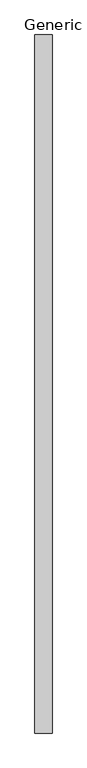
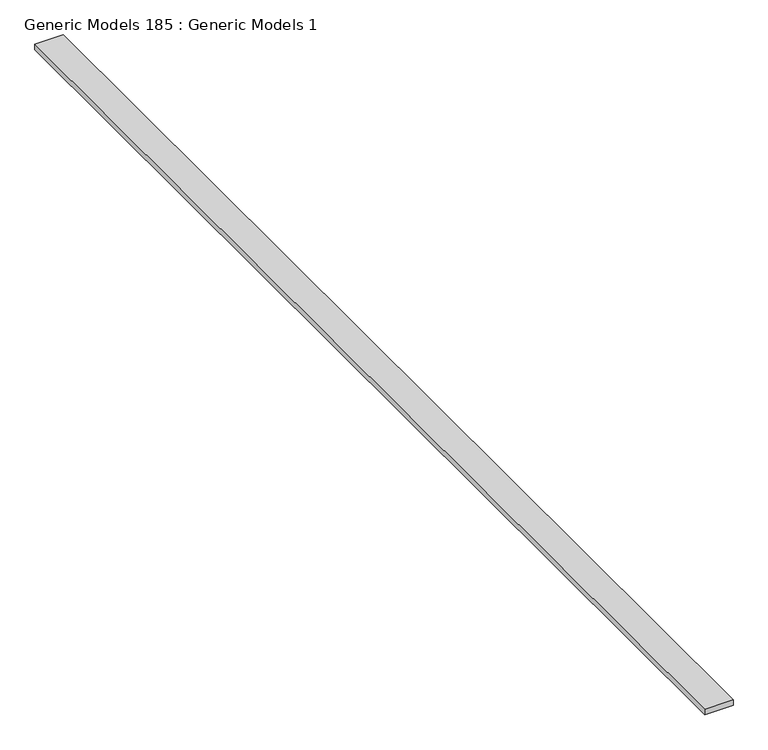
"""IFC4 building model written with IfcOpenShell, lengths in millimetres: proxy geometry, Generic Models 185 : Generic Models 1."""

import ifcopenshell
import ifcopenshell.guid

model = None  # the IFC model being written
_history = None  # IfcOwnerHistory: only IFC2X3 demands one
_inside = {}  # id of a spatial element -> (the spatial element, [elements in it])
_under = {}  # id of a project, library or spatial element -> (it, [spatial elements below it])
_declared = {}  # id of a project -> (the project, [libraries it declares])
_typed = {}  # id of a type object -> (the type object, [elements of that type])
_made_of = {}  # id of a material, layer set ... -> (it, [elements and type objects made of it])


def new_model(schema):
    """Start an empty IFC model of exactly this schema.

    Asked for "IFC4X3", IfcOpenShell would pick the latest addendum, in which some entities
    have other attributes; the version numbers below select the first issue.
    IFC2X3 requires an IfcOwnerHistory on every rooted entity: one is made here for all.
    """
    global model, _history
    if schema == "IFC4X3":
        model = ifcopenshell.file(schema_version=(4, 3, 0, 0))
    else:
        model = ifcopenshell.file(schema=schema)
    _inside.clear()
    _under.clear()
    _declared.clear()
    _typed.clear()
    _made_of.clear()
    _history = None
    if model.schema == "IFC2X3":
        org = make("IfcOrganization", Name="unknown")
        user = make(
            "IfcPersonAndOrganization",
            ThePerson=make("IfcPerson", FamilyName="unknown"),
            TheOrganization=org,
        )
        app = make(
            "IfcApplication",
            ApplicationDeveloper=org,
            Version="unknown",
            ApplicationFullName="unknown",
            ApplicationIdentifier="unknown",
        )
        _history = make(
            "IfcOwnerHistory",
            OwningUser=user,
            OwningApplication=app,
            ChangeAction="ADDED",
            CreationDate=0,
        )
    return model


def make(cls, **values):
    """One entity of the class cls with the attributes given. An attribute that is None is left unset."""
    return model.create_entity(
        cls, **{name: value for name, value in values.items() if value is not None}
    )


def rooted(cls, **values):
    """An entity with a GlobalId (a new one), such as an element, a storey or a relation."""
    return make(cls, GlobalId=ifcopenshell.guid.new(), OwnerHistory=_history, **values)


def si_unit(unit_type, name, prefix=None):
    """IfcSIUnit, for example si_unit("LENGTHUNIT", "METRE", prefix="MILLI")."""
    return make("IfcSIUnit", UnitType=unit_type, Prefix=prefix, Name=name)


def assignment(units):
    """IfcUnitAssignment: the units of a project."""
    return None if units is None else make("IfcUnitAssignment", Units=units)


def point(xyz):
    """IfcCartesianPoint."""
    return None if xyz is None else make("IfcCartesianPoint", Coordinates=xyz)


def direction(xyz):
    """IfcDirection."""
    return None if xyz is None else make("IfcDirection", DirectionRatios=xyz)


def frame(location, z_axis=None, x_axis=None):
    """IfcAxis2Placement3D, a coordinate frame: its origin and axes. An axis left out is left unset."""
    return make(
        "IfcAxis2Placement3D",
        Location=point(location),
        Axis=direction(z_axis),
        RefDirection=direction(x_axis),
    )


def origin():
    """The frame at (0, 0, 0) with its axes left unset."""
    return frame((0.0, 0.0, 0.0))


def place(relative_to, where):
    """IfcLocalPlacement: puts the frame where relative to a parent placement (None: the world)."""
    return make(
        "IfcLocalPlacement", PlacementRelTo=relative_to, RelativePlacement=where
    )


def context(
    kind, dimensions, precision=None, world=None, true_north=None, identifier=None
):
    """IfcGeometricRepresentationContext, for example the 3D "Model" context."""
    return make(
        "IfcGeometricRepresentationContext",
        ContextIdentifier=identifier,
        ContextType=kind,
        CoordinateSpaceDimension=dimensions,
        Precision=precision,
        WorldCoordinateSystem=world,
        TrueNorth=true_north,
    )


def project(units=None, contexts=None):
    """IfcProject with its units and contexts."""
    return rooted(
        "IfcProject",
        Name="project",
        RepresentationContexts=contexts,
        UnitsInContext=assignment(units),
    )


def spatial(cls, under=None, at=None, **own):
    """A site, building, storey or space (cls), placed at a placement, below another one or the project."""
    s = rooted(cls, ObjectPlacement=at, **own)
    if under is not None:
        _under.setdefault(under.id(), (under, []))[1].append(s)
    return s


def polyline(points):
    """IfcPolyline through the points."""
    return make("IfcPolyline", Points=[point(p) for p in points])


def outline(outer, holes=None, kind="AREA"):
    """IfcArbitraryClosedProfileDef: a profile drawn as a closed curve; with holes, ...WithVoids."""
    if holes is None:
        return make("IfcArbitraryClosedProfileDef", ProfileType=kind, OuterCurve=outer)
    return make(
        "IfcArbitraryProfileDefWithVoids",
        ProfileType=kind,
        OuterCurve=outer,
        InnerCurves=holes,
    )


def extrude(swept, where, along, depth):
    """IfcExtrudedAreaSolid: the profile swept, set in the frame where, extruded along a direction by depth."""
    return make(
        "IfcExtrudedAreaSolid",
        SweptArea=swept,
        Position=where,
        ExtrudedDirection=direction(along),
        Depth=depth,
    )


def shape(context_of_items, identifier, shape_type, items):
    """IfcShapeRepresentation: the items that make up one representation, for example the "Body"."""
    return make(
        "IfcShapeRepresentation",
        ContextOfItems=context_of_items,
        RepresentationIdentifier=identifier,
        RepresentationType=shape_type,
        Items=items,
    )


def source(mapping_origin, context_of_items, identifier, shape_type, items):
    """IfcRepresentationMap: a shape defined once, which mapped items show again and again."""
    return make(
        "IfcRepresentationMap",
        MappingOrigin=mapping_origin,
        MappedRepresentation=shape(context_of_items, identifier, shape_type, items),
    )


def transform(
    local_origin,
    x_axis=None,
    y_axis=None,
    z_axis=None,
    scale=None,
    scale2=None,
    scale3=None,
    uniform=True,
):
    """IfcCartesianTransformationOperator3D, or its non-uniform kind. x_axis, y_axis, z_axis: its Axis1, 2, 3."""
    if uniform:
        return make(
            "IfcCartesianTransformationOperator3D",
            Axis1=direction(x_axis),
            Axis2=direction(y_axis),
            LocalOrigin=point(local_origin),
            Scale=scale,
            Axis3=direction(z_axis),
        )
    return make(
        "IfcCartesianTransformationOperator3DnonUniform",
        Axis1=direction(x_axis),
        Axis2=direction(y_axis),
        LocalOrigin=point(local_origin),
        Scale=scale,
        Axis3=direction(z_axis),
        Scale2=scale2,
        Scale3=scale3,
    )


def mapped(mapping_source, mapping_target):
    """IfcMappedItem: shows the shape of a source again, moved by a transform."""
    return make(
        "IfcMappedItem", MappingSource=mapping_source, MappingTarget=mapping_target
    )


def made_of(thing, what):
    """Note that an element or type object is made of a material, layer set ...; save() writes the relation."""
    if what is not None:
        _made_of.setdefault(what.id(), (what, []))[1].append(thing)
    return thing


def element(
    cls,
    number,
    at=None,
    inside=None,
    cuts=None,
    type_object=None,
    material=None,
    context=None,
    identifier="Body",
    shape_type=None,
    held_by="IfcProductDefinitionShape",
    body=None,
    shapes=None,
    **own,
):
    """One element of the class cls, such as IfcWall. Its Tag is "e" and its number.

    at: its placement. inside: the storey or other place that contains it. cuts: it is an
    opening in that element (IfcRelVoidsElement). A single representation is given by context,
    identifier, shape_type and body (its items); several are given by shapes. held_by: the class
    of the entity that holds the representations. save() writes the other relations.
    """
    e = rooted(cls, Tag="e%d" % number, ObjectPlacement=at, **own)
    if body is not None:
        shapes = [shape(context, identifier, shape_type, body)]
    if shapes is not None:
        e.Representation = make(held_by, Representations=shapes)
    if inside is not None:
        _inside.setdefault(inside.id(), (inside, []))[1].append(e)
    if cuts is not None:
        rooted(
            "IfcRelVoidsElement", RelatingBuildingElement=cuts, RelatedOpeningElement=e
        )
    if type_object is not None:
        _typed.setdefault(type_object.id(), (type_object, []))[1].append(e)
    return made_of(e, material)


def aggregate(whole, parts):
    """IfcRelAggregates: a whole, such as a stair, and the parts it consists of."""
    return rooted("IfcRelAggregates", RelatingObject=whole, RelatedObjects=parts)


def save(model, path):
    """Write the relations noted so far, then the file.

    IfcRelAggregates (storeys below a building ...), IfcRelContainedInSpatialStructure (elements
    in a storey), IfcRelDefinesByType, IfcRelAssociatesMaterial and IfcRelDeclares: one each for
    every whole, place, type object, material and project.
    """
    for whole, parts in _under.values():
        aggregate(whole, parts)
    for where, things in _inside.values():
        rooted(
            "IfcRelContainedInSpatialStructure",
            RelatedElements=things,
            RelatingStructure=where,
        )
    for kind, things in _typed.values():
        rooted("IfcRelDefinesByType", RelatedObjects=things, RelatingType=kind)
    for what, things in _made_of.values():
        rooted("IfcRelAssociatesMaterial", RelatedObjects=things, RelatingMaterial=what)
    for by, libraries in _declared.values():
        rooted("IfcRelDeclares", RelatingContext=by, RelatedDefinitions=libraries)
    model.write(path)


def generic_models_185_generic_models_1_d53f1798(model_context):
    return source(origin(), model_context, "Body", "SweptSolid", [
        extrude(outline(polyline([(-5275.7536296, 7054.2769662), (-5091.6036296, 7054.2769662), (-5091.6036296, -464.1230338), (-5275.7536296, -464.1230338), (-5275.7536296, 7054.2769662)])), frame((0.0, 0.0, 126736.221), z_axis=(0.0, 0.0, 1.0), x_axis=(1.0, 0.0, 0.0)), (0.0, 0.0, 1.0), 38.1),
    ])


if __name__ == "__main__":
    model = new_model("IFC4")
    model_context = context("Model", 3, world=origin())
    ifc_project = project(units=[si_unit("LENGTHUNIT", "METRE", prefix="MILLI")], contexts=[model_context])
    site = spatial("IfcSite", under=ifc_project)
    building = spatial("IfcBuilding", under=site)
    placement = place(None, origin())
    generic_models_185_generic_models_1_shape = generic_models_185_generic_models_1_d53f1798(model_context)
    element("IfcBuildingElementProxy", 1, Name="Generic Models 185 : Generic Models 1", ObjectType="Generic Models 185 : Generic Models 1", at=placement, inside=building, context=model_context, shape_type="MappedRepresentation", body=[
        mapped(generic_models_185_generic_models_1_shape, transform((0.0, 0.0, 0.0), x_axis=(1.0, 0.0, 0.0), y_axis=(0.0, 1.0, 0.0), z_axis=(0.0, 0.0, 1.0))),
    ])
    save(model, "model.ifc")

# Revit data of these elements
# Element 1 (IfcBuildingElementProxy, "Generic Models 185 : Generic Models 1")
#   Materials on its faces: "_2X BLOCKING AS REQUIRED"
# Materials
#   "_2X BLOCKING AS REQUIRED": class "Generic", colour RGB 177 130 114, transparency 0, Cost = 0
